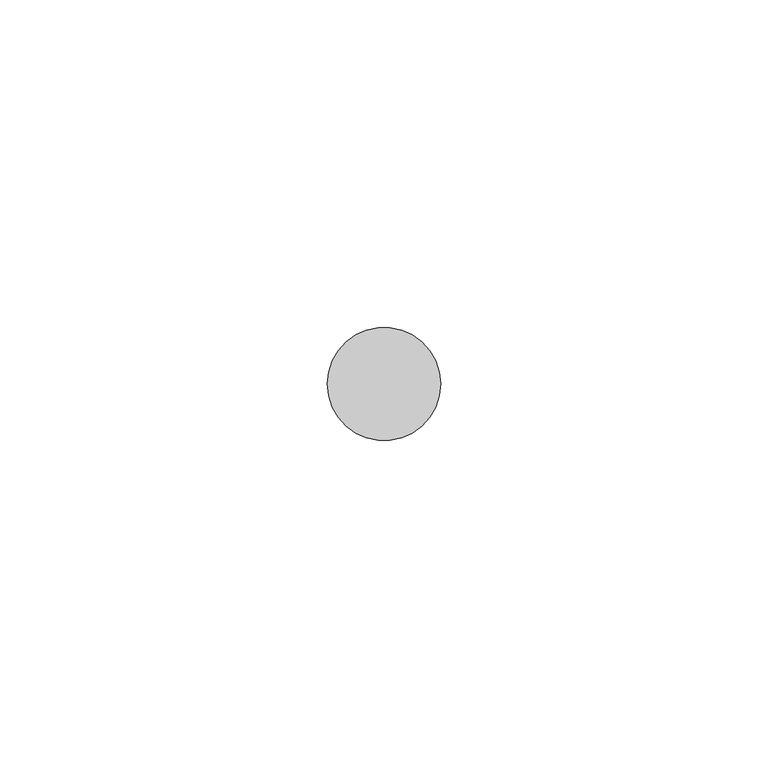
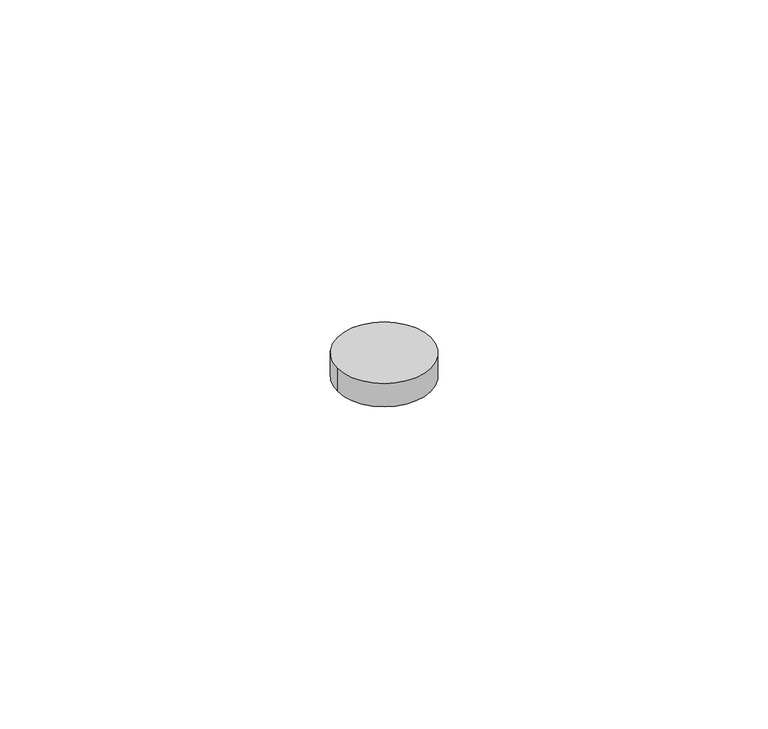
"""IFC4 building model written with IfcOpenShell, lengths in millimetres: proxy geometry, Hinge Pin Keeper7 : Hinge Pin Keeper."""

import ifcopenshell
import ifcopenshell.guid

model = None  # the IFC model being written
_history = None  # IfcOwnerHistory: only IFC2X3 demands one
_inside = {}  # id of a spatial element -> (the spatial element, [elements in it])
_under = {}  # id of a project, library or spatial element -> (it, [spatial elements below it])
_declared = {}  # id of a project -> (the project, [libraries it declares])
_typed = {}  # id of a type object -> (the type object, [elements of that type])
_made_of = {}  # id of a material, layer set ... -> (it, [elements and type objects made of it])


def new_model(schema):
    """Start an empty IFC model of exactly this schema.

    Asked for "IFC4X3", IfcOpenShell would pick the latest addendum, in which some entities
    have other attributes; the version numbers below select the first issue.
    IFC2X3 requires an IfcOwnerHistory on every rooted entity: one is made here for all.
    """
    global model, _history
    if schema == "IFC4X3":
        model = ifcopenshell.file(schema_version=(4, 3, 0, 0))
    else:
        model = ifcopenshell.file(schema=schema)
    _inside.clear()
    _under.clear()
    _declared.clear()
    _typed.clear()
    _made_of.clear()
    _history = None
    if model.schema == "IFC2X3":
        org = make("IfcOrganization", Name="unknown")
        user = make(
            "IfcPersonAndOrganization",
            ThePerson=make("IfcPerson", FamilyName="unknown"),
            TheOrganization=org,
        )
        app = make(
            "IfcApplication",
            ApplicationDeveloper=org,
            Version="unknown",
            ApplicationFullName="unknown",
            ApplicationIdentifier="unknown",
        )
        _history = make(
            "IfcOwnerHistory",
            OwningUser=user,
            OwningApplication=app,
            ChangeAction="ADDED",
            CreationDate=0,
        )
    return model


def make(cls, **values):
    """One entity of the class cls with the attributes given. An attribute that is None is left unset."""
    return model.create_entity(
        cls, **{name: value for name, value in values.items() if value is not None}
    )


def rooted(cls, **values):
    """An entity with a GlobalId (a new one), such as an element, a storey or a relation."""
    return make(cls, GlobalId=ifcopenshell.guid.new(), OwnerHistory=_history, **values)


def si_unit(unit_type, name, prefix=None):
    """IfcSIUnit, for example si_unit("LENGTHUNIT", "METRE", prefix="MILLI")."""
    return make("IfcSIUnit", UnitType=unit_type, Prefix=prefix, Name=name)


def assignment(units):
    """IfcUnitAssignment: the units of a project."""
    return None if units is None else make("IfcUnitAssignment", Units=units)


def point(xyz):
    """IfcCartesianPoint."""
    return None if xyz is None else make("IfcCartesianPoint", Coordinates=xyz)


def direction(xyz):
    """IfcDirection."""
    return None if xyz is None else make("IfcDirection", DirectionRatios=xyz)


def frame(location, z_axis=None, x_axis=None):
    """IfcAxis2Placement3D, a coordinate frame: its origin and axes. An axis left out is left unset."""
    return make(
        "IfcAxis2Placement3D",
        Location=point(location),
        Axis=direction(z_axis),
        RefDirection=direction(x_axis),
    )


def frame_2d(location, x_axis=None):
    """IfcAxis2Placement2D, a coordinate frame in the plane: its origin and x axis."""
    return make(
        "IfcAxis2Placement2D", Location=point(location), RefDirection=direction(x_axis)
    )


def origin():
    """The frame at (0, 0, 0) with its axes left unset."""
    return frame((0.0, 0.0, 0.0))


def place(relative_to, where):
    """IfcLocalPlacement: puts the frame where relative to a parent placement (None: the world)."""
    return make(
        "IfcLocalPlacement", PlacementRelTo=relative_to, RelativePlacement=where
    )


def context(
    kind, dimensions, precision=None, world=None, true_north=None, identifier=None
):
    """IfcGeometricRepresentationContext, for example the 3D "Model" context."""
    return make(
        "IfcGeometricRepresentationContext",
        ContextIdentifier=identifier,
        ContextType=kind,
        CoordinateSpaceDimension=dimensions,
        Precision=precision,
        WorldCoordinateSystem=world,
        TrueNorth=true_north,
    )


def project(units=None, contexts=None):
    """IfcProject with its units and contexts."""
    return rooted(
        "IfcProject",
        Name="project",
        RepresentationContexts=contexts,
        UnitsInContext=assignment(units),
    )


def spatial(cls, under=None, at=None, **own):
    """A site, building, storey or space (cls), placed at a placement, below another one or the project."""
    s = rooted(cls, ObjectPlacement=at, **own)
    if under is not None:
        _under.setdefault(under.id(), (under, []))[1].append(s)
    return s


def circle_curve(where, radius):
    """IfcCircle in the frame where."""
    return make("IfcCircle", Position=where, Radius=radius)


def trimmed(basis, trim1, trim2, sense, master):
    """IfcTrimmedCurve: the piece of a basis curve between two trims."""
    return make(
        "IfcTrimmedCurve",
        BasisCurve=basis,
        Trim1=trim1,
        Trim2=trim2,
        SenseAgreement=sense,
        MasterRepresentation=master,
    )


def segment(curve, same_sense, transition):
    """IfcCompositeCurveSegment."""
    return make(
        "IfcCompositeCurveSegment",
        Transition=transition,
        SameSense=same_sense,
        ParentCurve=curve,
    )


def composite_curve(segments, self_intersect=None):
    """IfcCompositeCurve: segments joined end to end."""
    return make("IfcCompositeCurve", Segments=segments, SelfIntersect=self_intersect)


def outline(outer, holes=None, kind="AREA"):
    """IfcArbitraryClosedProfileDef: a profile drawn as a closed curve; with holes, ...WithVoids."""
    if holes is None:
        return make("IfcArbitraryClosedProfileDef", ProfileType=kind, OuterCurve=outer)
    return make(
        "IfcArbitraryProfileDefWithVoids",
        ProfileType=kind,
        OuterCurve=outer,
        InnerCurves=holes,
    )


def extrude(swept, where, along, depth):
    """IfcExtrudedAreaSolid: the profile swept, set in the frame where, extruded along a direction by depth."""
    return make(
        "IfcExtrudedAreaSolid",
        SweptArea=swept,
        Position=where,
        ExtrudedDirection=direction(along),
        Depth=depth,
    )


def shape(context_of_items, identifier, shape_type, items):
    """IfcShapeRepresentation: the items that make up one representation, for example the "Body"."""
    return make(
        "IfcShapeRepresentation",
        ContextOfItems=context_of_items,
        RepresentationIdentifier=identifier,
        RepresentationType=shape_type,
        Items=items,
    )


def source(mapping_origin, context_of_items, identifier, shape_type, items):
    """IfcRepresentationMap: a shape defined once, which mapped items show again and again."""
    return make(
        "IfcRepresentationMap",
        MappingOrigin=mapping_origin,
        MappedRepresentation=shape(context_of_items, identifier, shape_type, items),
    )


def transform(
    local_origin,
    x_axis=None,
    y_axis=None,
    z_axis=None,
    scale=None,
    scale2=None,
    scale3=None,
    uniform=True,
):
    """IfcCartesianTransformationOperator3D, or its non-uniform kind. x_axis, y_axis, z_axis: its Axis1, 2, 3."""
    if uniform:
        return make(
            "IfcCartesianTransformationOperator3D",
            Axis1=direction(x_axis),
            Axis2=direction(y_axis),
            LocalOrigin=point(local_origin),
            Scale=scale,
            Axis3=direction(z_axis),
        )
    return make(
        "IfcCartesianTransformationOperator3DnonUniform",
        Axis1=direction(x_axis),
        Axis2=direction(y_axis),
        LocalOrigin=point(local_origin),
        Scale=scale,
        Axis3=direction(z_axis),
        Scale2=scale2,
        Scale3=scale3,
    )


def mapped(mapping_source, mapping_target):
    """IfcMappedItem: shows the shape of a source again, moved by a transform."""
    return make(
        "IfcMappedItem", MappingSource=mapping_source, MappingTarget=mapping_target
    )


def made_of(thing, what):
    """Note that an element or type object is made of a material, layer set ...; save() writes the relation."""
    if what is not None:
        _made_of.setdefault(what.id(), (what, []))[1].append(thing)
    return thing


def element(
    cls,
    number,
    at=None,
    inside=None,
    cuts=None,
    type_object=None,
    material=None,
    context=None,
    identifier="Body",
    shape_type=None,
    held_by="IfcProductDefinitionShape",
    body=None,
    shapes=None,
    **own,
):
    """One element of the class cls, such as IfcWall. Its Tag is "e" and its number.

    at: its placement. inside: the storey or other place that contains it. cuts: it is an
    opening in that element (IfcRelVoidsElement). A single representation is given by context,
    identifier, shape_type and body (its items); several are given by shapes. held_by: the class
    of the entity that holds the representations. save() writes the other relations.
    """
    e = rooted(cls, Tag="e%d" % number, ObjectPlacement=at, **own)
    if body is not None:
        shapes = [shape(context, identifier, shape_type, body)]
    if shapes is not None:
        e.Representation = make(held_by, Representations=shapes)
    if inside is not None:
        _inside.setdefault(inside.id(), (inside, []))[1].append(e)
    if cuts is not None:
        rooted(
            "IfcRelVoidsElement", RelatingBuildingElement=cuts, RelatedOpeningElement=e
        )
    if type_object is not None:
        _typed.setdefault(type_object.id(), (type_object, []))[1].append(e)
    return made_of(e, material)


def aggregate(whole, parts):
    """IfcRelAggregates: a whole, such as a stair, and the parts it consists of."""
    return rooted("IfcRelAggregates", RelatingObject=whole, RelatedObjects=parts)


def save(model, path):
    """Write the relations noted so far, then the file.

    IfcRelAggregates (storeys below a building ...), IfcRelContainedInSpatialStructure (elements
    in a storey), IfcRelDefinesByType, IfcRelAssociatesMaterial and IfcRelDeclares: one each for
    every whole, place, type object, material and project.
    """
    for whole, parts in _under.values():
        aggregate(whole, parts)
    for where, things in _inside.values():
        rooted(
            "IfcRelContainedInSpatialStructure",
            RelatedElements=things,
            RelatingStructure=where,
        )
    for kind, things in _typed.values():
        rooted("IfcRelDefinesByType", RelatedObjects=things, RelatingType=kind)
    for what, things in _made_of.values():
        rooted("IfcRelAssociatesMaterial", RelatedObjects=things, RelatingMaterial=what)
    for by, libraries in _declared.values():
        rooted("IfcRelDeclares", RelatingContext=by, RelatedDefinitions=libraries)
    model.write(path)


def generic_models_10b8f884(model_context):
    return source(origin(), model_context, "Body", "SweptSolid", [
        extrude(outline(composite_curve([segment(trimmed(circle_curve(frame_2d((587319.1320739, -534100.7049841)), 8.6534625), [point((587310.4786114, -534100.7049841))], [point((587327.7855364, -534100.7049841))], False, "CARTESIAN"), True, "CONTINUOUS"), segment(trimmed(circle_curve(frame_2d((587319.1320739, -534100.7049841)), 8.6534625), [point((587327.7855364, -534100.7049841))], [point((587310.4786114, -534100.7049841))], False, "CARTESIAN"), True, "CONTINUOUS")], self_intersect=False)), frame((0.0, 0.0, 2084.5859375), z_axis=(0.0, 0.0, 1.0), x_axis=(1.0, 0.0, 0.0)), (0.0, 0.0, 1.0), 4.5640625),
    ])


if __name__ == "__main__":
    model = new_model("IFC4")
    model_context = context("Model", 3, world=origin())
    ifc_project = project(units=[si_unit("LENGTHUNIT", "METRE", prefix="MILLI")], contexts=[model_context])
    site = spatial("IfcSite", under=ifc_project)
    building = spatial("IfcBuilding", under=site)
    placement = place(None, origin())
    generic_models_shape = generic_models_10b8f884(model_context)
    element("IfcBuildingElementProxy", 1, Name="Hinge Pin Keeper7 : Hinge Pin Keeper", ObjectType="Hinge Pin Keeper7 : Hinge Pin Keeper", at=placement, inside=building, context=model_context, shape_type="MappedRepresentation", body=[
        mapped(generic_models_shape, transform((0.0, 0.0, 0.0), x_axis=(1.0, 0.0, 0.0), y_axis=(0.0, 1.0, 0.0), z_axis=(0.0, 0.0, 1.0))),
    ])
    save(model, "model.ifc")

# Revit data of these elements
# Element 1 (IfcBuildingElementProxy, "Hinge Pin Keeper7 : Hinge Pin Keeper")
#   Materials on its faces: "6\"X6\" WELD-ON STL BUTT HINGE"
# Materials
#   "6\"X6\" WELD-ON STL BUTT HINGE": class "Metal", colour RGB 189 187 185, transparency 0, Description = "Carbon steel", Cost = 0
